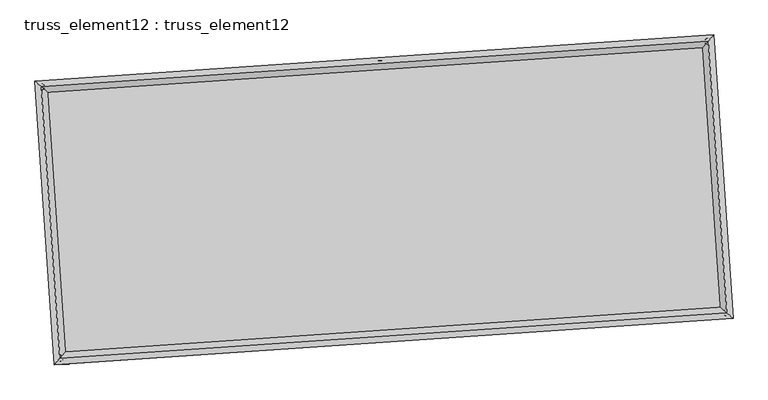
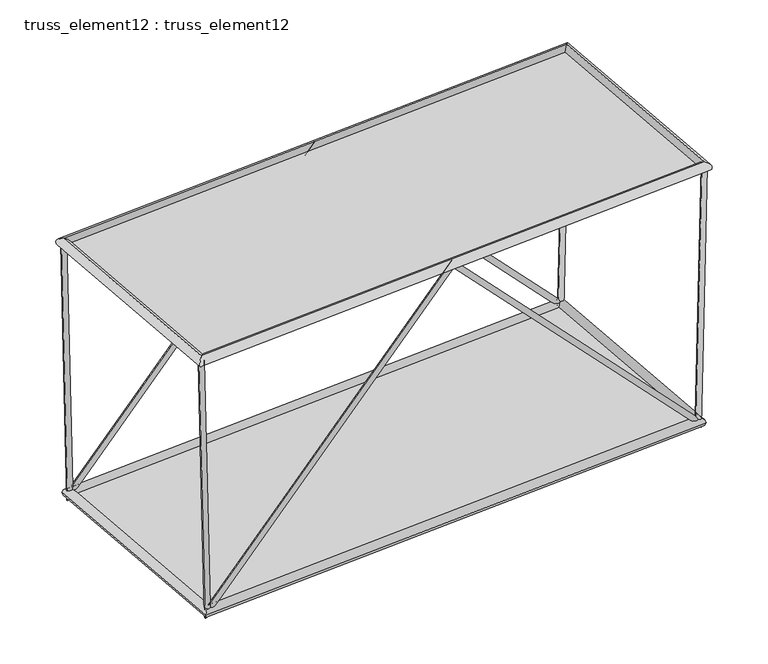
"""IFC4 building model written with IfcOpenShell, lengths in millimetres: plate geometry, truss_element12 : truss_element12."""

from ifc_helpers import new_model, si_unit, frame, origin, origin_with_axes, place, context, project, spatial, polyline, circle_curve, ellipse_curve, outline, extrude, source, transform, mapped, element, save
from ifc_brep_helpers import plane_surface, cylinder_surface, advanced_brep


def truss_element12_truss_element12_a892e973(model_context):
    return source(origin(), model_context, "Body", "SolidModel", [
        advanced_brep(
        [(-3781.9001647, 2268.2490038, 4999.7954617), (-3880.9761734, 2254.8896434, 4997.4562298), (-3667.764278, 2276.0314961, 121.2292813), (-3761.2226048, 2263.055184, -121.2292813), (1063.7843207, 2598.6578087, 5070.7379408), (1064.2315522, 2592.0845597, 4926.5107211), (5795.2062001, 2921.2754808, 121.228402), (5889.5547769, 2921.1050077, -121.228402), (5909.4678674, 2929.0665496, 4999.7937205), (6009.4402165, 2929.2795401, 4997.4519118)],
        [
            (0, 1, circle_curve(frame((-3831.4381691, 2261.5693236, 4998.6258457), z_axis=(-0.02338894552682542, -0.0015948032857686179, 0.9997251691488132), x_axis=(-0.13359419431199426, 0.9910349164502389, -0.0015445460813113196)), 50.0)),
            (1, 0, circle_curve(frame((-3831.4381691, 2261.5693236, 4998.6258457), z_axis=(-0.02338894552682542, -0.0015948032857686179, 0.9997251691488132), x_axis=(-0.13359419431199426, 0.9910349164502389, -0.0015445460813113196)), 50.0)),
            (0, 2),
            (2, 3, ellipse_curve(frame((-3714.4934414, 2269.54334, 0.0), z_axis=(-0.9300590534640556, -0.06341719137026212, 0.36189558840672914), x_axis=(0.3610572196661413, 0.024619119302049103, 0.9322186348125354)), 130.3269965, 50.0)),
            (3, 1),
            (3, 2, ellipse_curve(frame((-3714.4934414, 2269.54334, 0.0), z_axis=(-0.9300590534640556, -0.06341719137026212, 0.36189558840672914), x_axis=(0.3610572196661413, 0.024619119302049103, 0.9322186348125354)), 130.3269965, 50.0)),
            (2, 4),
            (4, 5, ellipse_curve(frame((1064.0079364, 2595.3711842, 4998.6243309), z_axis=(-0.997683396052257, -0.06802823822715924, 6.733807032577008e-06), x_axis=(-6.718207468772972e-06, -4.580890289962869e-07, -0.9999999999773278)), 72.2706352, 50.0)),
            (5, 3),
            (5, 4, ellipse_curve(frame((1064.0079364, 2595.3711842, 4998.6243309), z_axis=(-0.997683396052257, -0.06802823822715924, 6.733807032577008e-06), x_axis=(-6.718207468772972e-06, -4.580890289962869e-07, -0.9999999999773278)), 72.2706352, 50.0)),
            (4, 6),
            (6, 7, ellipse_curve(frame((5842.3804885, 2921.1902443, 0.0), z_axis=(-0.9300661480063922, -0.06341767512013534, -0.3618772703761719), x_axis=(-0.3610389440712053, -0.024617873158702383, 0.9322257458282791)), 130.3250571, 50.0)),
            (7, 5),
            (7, 6, ellipse_curve(frame((5842.3804885, 2921.1902443, 0.0), z_axis=(-0.9300661480063922, -0.06341767512013534, -0.3618772703761719), x_axis=(-0.3610389440712053, -0.024617873158702383, 0.9322257458282791)), 130.3250571, 50.0)),
            (8, 9, circle_curve(frame((5959.4540419, 2929.1730448, 4998.6228161), z_axis=(0.02341471068854339, 0.0015965601142037436, 0.9997245632268789), x_axis=(-0.0021667064549673746, 0.9999964572445558, -0.0015462475466263355)), 50.0)),
            (9, 8, circle_curve(frame((5959.4540419, 2929.1730448, 4998.6228161), z_axis=(0.02341471068854339, 0.0015965601142037436, 0.9997245632268789), x_axis=(-0.0021667064549673746, 0.9999964572445558, -0.0015462475466263355)), 50.0)),
            (6, 8),
            (9, 7),
        ],
        [
            plane_surface(frame((-3831.4381691, 2311.56926, 4998.7056077), z_axis=(-0.023388945526825605, -0.0015948032857737312, 0.9997251691488132), x_axis=(0.9997264411963621, -3.731097392201122e-05, 0.023388915766833666))),
            cylinder_surface(frame((-3831.4381691, 2261.5693236, 4998.6258457), z_axis=(-0.02338894552682542, -0.0015948032857686179, 0.9997251691488132), x_axis=(-0.13359419431199426, 0.9910349164502389, -0.0015445460813113196)), 50.0),
            cylinder_surface(frame((-3714.4934414, 2269.54334, 0.0), z_axis=(-0.6902460485200175, -0.04706525417770467, -0.7220424186650602), x_axis=(-0.0204192616913266, 0.9987518848874466, -0.04558208184971222)), 50.0),
            cylinder_surface(frame((1064.0079364, 2595.3711842, 4998.6243309), z_axis=(-0.6902363467958805, -0.04706459265401546, 0.7220517361520492), x_axis=(-0.11534221170273892, 0.9922794497620825, -0.045581441172688954)), 50.0),
            plane_surface(frame((5959.4540419, 2879.1731086, 4998.702666), z_axis=(0.02341471068854475, 0.0015965601141989436, 0.999724563226879), x_axis=(0.9997258380793066, -3.739324497509243e-05, -0.023414680830057922))),
            cylinder_surface(frame((5842.3804885, 2921.1902443, 0.0), z_axis=(-0.02341471068854339, -0.0015965601142037436, -0.9997245632268789), x_axis=(-0.0021667064549673746, 0.9999964572445558, -0.0015462475466263355)), 50.0),
        ],
        [
            (0, [[1, 2]]),
            (1, [[-1, 3, 4, 5]]),
            (1, [[-2, -5, 6, -3]]),
            (2, [[-4, 7, 8, 9]]),
            (2, [[-6, -9, 10, -7]]),
            (3, [[-8, 11, 12, 13]]),
            (3, [[-10, -13, 14, -11]]),
            (4, [[15, 16]]),
            (5, [[-12, 17, -16, 18]]),
            (5, [[-14, -18, -15, -17]]),
        ],
    ),
        advanced_brep(
        [(-3509.7872118, -1722.4845805, 4999.7954617), (-3608.8632204, -1735.8439409, 4997.4562298), (-3395.6513251, -1714.7020882, 121.2292813), (-3489.1096519, -1727.6784003, -121.2292813), (1335.8972737, -1392.0757756, 5070.7379408), (1336.3445051, -1398.6490246, 4926.5107211), (6067.319153, -1069.4581035, 121.228402), (6161.6677299, -1069.6285766, -121.228402), (6181.5808204, -1061.6670347, 4999.7937205), (6281.5531694, -1061.4540442, 4997.4519118)],
        [
            (0, 1, circle_curve(frame((-3559.3252161, -1729.1642607, 4998.6258457), z_axis=(-0.023388945526825546, -0.0015948032857685606, 0.9997251691488132), x_axis=(-0.1335941943119938, 0.991034916450239, -0.0015445460813113816)), 50.0)),
            (1, 0, circle_curve(frame((-3559.3252161, -1729.1642607, 4998.6258457), z_axis=(-0.023388945526825546, -0.0015948032857685606, 0.9997251691488132), x_axis=(-0.1335941943119938, 0.991034916450239, -0.0015445460813113816)), 50.0)),
            (0, 2),
            (2, 3, ellipse_curve(frame((-3442.3804885, -1721.1902443, 0.0), z_axis=(-0.9300590534640557, -0.06341719137026187, 0.36189558840672914), x_axis=(0.36105721966614135, 0.024619119302049068, 0.9322186348125354)), 130.3269965, 50.0)),
            (3, 1),
            (3, 2, ellipse_curve(frame((-3442.3804885, -1721.1902443, 0.0), z_axis=(-0.9300590534640557, -0.06341719137026187, 0.36189558840672914), x_axis=(0.36105721966614135, 0.024619119302049068, 0.9322186348125354)), 130.3269965, 50.0)),
            (2, 4),
            (4, 5, ellipse_curve(frame((1336.1208894, -1395.3624001, 4998.6243309), z_axis=(-0.997683396052257, -0.06802823822715906, 6.733807032737481e-06), x_axis=(-6.718207468926731e-06, -4.580890289866768e-07, -0.9999999999773278)), 72.2706352, 50.0)),
            (5, 3),
            (5, 4, ellipse_curve(frame((1336.1208894, -1395.3624001, 4998.6243309), z_axis=(-0.997683396052257, -0.06802823822715906, 6.733807032737481e-06), x_axis=(-6.718207468926731e-06, -4.580890289866768e-07, -0.9999999999773278)), 72.2706352, 50.0)),
            (4, 6),
            (6, 7, ellipse_curve(frame((6114.4934414, -1069.54334, 0.0), z_axis=(-0.9300661480063922, -0.06341767512013499, -0.36187727037617134), x_axis=(-0.36103894407120507, -0.024617873158702393, 0.9322257458282792)), 130.3250571, 50.0)),
            (7, 5),
            (7, 6, ellipse_curve(frame((6114.4934414, -1069.54334, 0.0), z_axis=(-0.9300661480063922, -0.06341767512013499, -0.36187727037617134), x_axis=(-0.36103894407120507, -0.024617873158702393, 0.9322257458282792)), 130.3250571, 50.0)),
            (8, 9, circle_curve(frame((6231.5669949, -1061.5605395, 4998.6228161), z_axis=(0.023414710688543654, 0.0015965601142036118, 0.9997245632268787), x_axis=(-0.002166706454967089, 0.9999964572445559, -0.0015462475466262102)), 50.0)),
            (9, 8, circle_curve(frame((6231.5669949, -1061.5605395, 4998.6228161), z_axis=(0.023414710688543654, 0.0015965601142036118, 0.9997245632268787), x_axis=(-0.002166706454967089, 0.9999964572445559, -0.0015462475466262102)), 50.0)),
            (6, 8),
            (9, 7),
        ],
        [
            plane_surface(frame((-3559.3252161, -1679.1643243, 4998.7056077), z_axis=(-0.023388945526825605, -0.0015948032857737268, 0.9997251691488132), x_axis=(0.9997264411963621, -3.731097392201122e-05, 0.023388915766833666))),
            cylinder_surface(frame((-3559.3252161, -1729.1642607, 4998.6258457), z_axis=(-0.023388945526825546, -0.0015948032857685606, 0.9997251691488132), x_axis=(-0.1335941943119938, 0.991034916450239, -0.0015445460813113816)), 50.0),
            cylinder_surface(frame((-3442.3804885, -1721.1902443, 0.0), z_axis=(-0.6902460485200175, -0.04706525417770453, -0.7220424186650602), x_axis=(-0.020419261691326598, 0.9987518848874467, -0.04558208184971204)), 50.0),
            cylinder_surface(frame((1336.1208894, -1395.3624001, 4998.6243309), z_axis=(-0.6902363467958806, -0.047064592654015365, 0.7220517361520495), x_axis=(-0.11534221170273865, 0.9922794497620827, -0.0455814411726888)), 50.0),
            plane_surface(frame((6231.5669949, -1111.5604757, 4998.702666), z_axis=(0.02341471068854475, 0.0015965601141989436, 0.999724563226879), x_axis=(0.9997258380793066, -3.739324497464834e-05, -0.023414680830057922))),
            cylinder_surface(frame((6114.4934414, -1069.54334, 0.0), z_axis=(-0.023414710688543658, -0.0015965601142036122, -0.999724563226879), x_axis=(-0.002166706454967089, 0.9999964572445559, -0.0015462475466262102)), 50.0),
        ],
        [
            (0, [[1, 2]]),
            (1, [[-1, 3, 4, 5]]),
            (1, [[-2, -5, 6, -3]]),
            (2, [[-4, 7, 8, 9]]),
            (2, [[-6, -9, 10, -7]]),
            (3, [[-8, 11, 12, 13]]),
            (3, [[-10, -13, 14, -11]]),
            (4, [[15, 16]]),
            (5, [[-12, 17, -16, 18]]),
            (5, [[-14, -18, -15, -17]]),
        ],
    ),
        advanced_brep(
        [(-3559.3260024, -1729.1651321, 4908.6258457), (-3559.3244299, -1729.1633893, 5088.6258457), (-3831.4372718, 2261.568567, 5088.6258457), (-3831.4390663, 2261.5700802, 4908.6258457), (5959.4533112, 2929.1721772, 5088.6228161), (5959.4547727, 2929.1739124, 4908.6228161), (6231.5661531, -1061.5597791, 5088.6228161), (6231.5678367, -1061.5612999, 4908.6228161)],
        [
            (0, 1, ellipse_curve(frame((-3559.3252161, -1729.1642607, 4998.6258457), z_axis=(-0.7535719234054201, 0.6573654662780878, 2.1829417809630158e-07), x_axis=(-0.6573654662780518, -0.7535719234054518, 2.182941780963455e-07)), 127.2792206, 90.0)),
            (1, 2),
            (2, 3, ellipse_curve(frame((-3831.4381691, 2261.5693236, 4998.6258457), z_axis=(-0.6573654662780518, -0.7535719234054514, 2.1829417809638662e-07), x_axis=(0.7535719234054199, -0.6573654662780882, -2.1829417809634269e-07)), 127.2792206, 90.0)),
            (3, 0),
            (1, 0, ellipse_curve(frame((-3559.3252161, -1729.1642607, 4998.6258457), z_axis=(-0.7535719234054201, 0.6573654662780878, 2.1829417809630158e-07), x_axis=(-0.6573654662780518, -0.7535719234054518, 2.182941780963455e-07)), 127.2792206, 90.0)),
            (3, 2, ellipse_curve(frame((-3831.4381691, 2261.5693236, 4998.6258457), z_axis=(-0.6573654662780518, -0.7535719234054514, 2.1829417809638662e-07), x_axis=(0.7535719234054199, -0.6573654662780882, -2.1829417809634269e-07)), 127.2792206, 90.0)),
            (2, 4),
            (4, 5, ellipse_curve(frame((5959.4540419, 2929.1730448, 4998.6228161), z_axis=(-0.7535719234054205, 0.6573654662780875, 2.1829417809638398e-07), x_axis=(-0.6573654662780517, -0.7535719234054518, 2.182941780963455e-07)), 127.2792206, 90.0)),
            (5, 3),
            (5, 4, ellipse_curve(frame((5959.4540419, 2929.1730448, 4998.6228161), z_axis=(-0.7535719234054205, 0.6573654662780875, 2.1829417809638398e-07), x_axis=(-0.6573654662780517, -0.7535719234054518, 2.182941780963455e-07)), 127.2792206, 90.0)),
            (4, 6),
            (6, 7, ellipse_curve(frame((6231.5669949, -1061.5605395, 4998.6228161), z_axis=(0.6573654662780518, 0.7535719234054516, -2.182941780963044e-07), x_axis=(-0.7535719234054203, 0.6573654662780877, 2.1829417809634276e-07)), 127.2792206, 90.0)),
            (7, 5),
            (7, 6, ellipse_curve(frame((6231.5669949, -1061.5605395, 4998.6228161), z_axis=(0.6573654662780518, 0.7535719234054516, -2.182941780963044e-07), x_axis=(-0.7535719234054203, 0.6573654662780877, 2.1829417809634276e-07)), 127.2792206, 90.0)),
            (6, 1),
            (0, 7),
        ],
        [
            cylinder_surface(frame((-3559.3252161, -1729.1642607, 4998.6258457), z_axis=(0.068028238228695, -0.997683396074877, 0.0), x_axis=(-0.9976833960310403, -0.06802823822570593, 9.37427355396154e-06)), 90.0),
            cylinder_surface(frame((-3831.4381691, 2261.5693236, 4998.6258457), z_axis=(-0.9976833960748295, -0.06802823822869196, 3.0871458725096684e-07), x_axis=(-0.06802823822310758, 0.9976833960340704, 9.065558966723289e-06)), 90.0),
            cylinder_surface(frame((5959.4540419, 2929.1730448, 4998.6228161), z_axis=(-0.06802823822869553, 0.9976833960748772, 0.0), x_axis=(0.9976833960366247, 0.06802823822608724, 8.75684437948504e-06)), 90.0),
            cylinder_surface(frame((6231.5669949, -1061.5605395, 4998.6228161), z_axis=(0.9976833960748296, 0.06802823822869167, -3.0871458725090866e-07), x_axis=(0.06802823822869167, -0.9976833960336897, 9.065558966723292e-06)), 90.0),
        ],
        [
            (0, [[1, 2, 3, 4]]),
            (0, [[5, -4, 6, -2]]),
            (1, [[-3, 7, 8, 9]]),
            (1, [[-6, -9, 10, -7]]),
            (2, [[-8, 11, 12, 13]]),
            (2, [[-10, -13, 14, -11]]),
            (3, [[-12, 15, -1, 16]]),
            (3, [[-14, -16, -5, -15]]),
        ],
    ),
        advanced_brep(
        [(-3358.7115243, -1625.2761972, 0.0), (-3526.0494527, -1817.1042913, 0.0), (-3810.4074885, 2353.2123043, 0.0), (-3618.5793943, 2185.8743758, 0.0), (5926.0494527, 3017.1042913, 0.0), (5758.7115243, 2825.2761972, 0.0), (6210.4074885, -1153.2123043, 0.0), (6018.5793943, -985.8743758, 0.0)],
        [
            (0, 1, ellipse_curve(frame((-3442.3804885, -1721.1902443, 0.0), z_axis=(-0.7535719234054582, 0.6573654662780805, 0.0), x_axis=(-0.6573654662780803, -0.7535719234054584, 0.0)), 127.2792206, 90.0)),
            (1, 2),
            (2, 3, ellipse_curve(frame((-3714.4934414, 2269.54334, 0.0), z_axis=(-0.6573654662780803, -0.7535719234054584, 0.0), x_axis=(0.7535719234054584, -0.6573654662780801, 0.0)), 127.2792206, 90.0)),
            (3, 0),
            (1, 0, ellipse_curve(frame((-3442.3804885, -1721.1902443, 0.0), z_axis=(-0.7535719234054582, 0.6573654662780805, 0.0), x_axis=(-0.6573654662780803, -0.7535719234054584, 0.0)), 127.2792206, 90.0)),
            (3, 2, ellipse_curve(frame((-3714.4934414, 2269.54334, 0.0), z_axis=(-0.6573654662780803, -0.7535719234054584, 0.0), x_axis=(0.7535719234054584, -0.6573654662780801, 0.0)), 127.2792206, 90.0)),
            (2, 4),
            (4, 5, ellipse_curve(frame((5842.3804885, 2921.1902443, 0.0), z_axis=(-0.7535719234054583, 0.6573654662780803, 0.0), x_axis=(-0.6573654662780803, -0.7535719234054583, 0.0)), 127.2792206, 90.0)),
            (5, 3),
            (5, 4, ellipse_curve(frame((5842.3804885, 2921.1902443, 0.0), z_axis=(-0.7535719234054583, 0.6573654662780803, 0.0), x_axis=(-0.6573654662780803, -0.7535719234054583, 0.0)), 127.2792206, 90.0)),
            (4, 6),
            (6, 7, ellipse_curve(frame((6114.4934414, -1069.54334, 0.0), z_axis=(0.6573654662780806, 0.7535719234054582, 0.0), x_axis=(-0.7535719234054582, 0.6573654662780806, 0.0)), 127.2792206, 90.0)),
            (7, 5),
            (7, 6, ellipse_curve(frame((6114.4934414, -1069.54334, 0.0), z_axis=(0.6573654662780806, 0.7535719234054582, 0.0), x_axis=(-0.7535719234054582, 0.6573654662780806, 0.0)), 127.2792206, 90.0)),
            (6, 1),
            (0, 7),
        ],
        [
            cylinder_surface(frame((-3442.3804885, -1721.1902443, 0.0), z_axis=(0.06802823822870183, -0.9976833960748765, 0.0), x_axis=(-0.9976833960748765, -0.06802823822870183, 0.0)), 90.0),
            cylinder_surface(frame((-3714.4934414, 2269.54334, 0.0), z_axis=(-0.9976833960748765, -0.068028238228702, 0.0), x_axis=(-0.068028238228702, 0.9976833960748765, 0.0)), 90.0),
            cylinder_surface(frame((5842.3804885, 2921.1902443, 0.0), z_axis=(-0.06802823822870174, 0.9976833960748765, 0.0), x_axis=(0.9976833960748765, 0.06802823822870174, 0.0)), 90.0),
            cylinder_surface(frame((6114.4934414, -1069.54334, 0.0), z_axis=(0.9976833960748768, 0.06802823822870133, 0.0), x_axis=(0.06802823822870133, -0.9976833960748768, 0.0)), 90.0),
        ],
        [
            (0, [[1, 2, 3, 4]]),
            (0, [[5, -4, 6, -2]]),
            (1, [[-3, 7, 8, 9]]),
            (1, [[-6, -9, 10, -7]]),
            (2, [[-8, 11, 12, 13]]),
            (2, [[-10, -13, 14, -11]]),
            (3, [[-12, 15, -1, 16]]),
            (3, [[-14, -16, -5, -15]]),
        ],
    ),
        extrude(outline(polyline([(-3442.3804885, -1721.1902443), (-3714.4934414, 2269.54334), (5842.3804885, 2921.1902443), (6114.4934414, -1069.54334), (-3442.3804885, -1721.1902443)])), origin_with_axes(), (0.0, 0.0, 1.0), 20.0),
        extrude(outline(polyline([(-2000.0000001, 4906.8132483), (2000.0, 4906.8132484), (2000.0, -4906.8132483), (-2000.0000001, -4906.8132484), (-2000.0000001, 4906.8132483)])), frame((1200.0644129, 600.0043921, 4998.6243309), z_axis=(3.0799941782636943e-07, 2.1001309486182012e-08, 0.9999999999999525), x_axis=(-0.06802823822870138, 0.9976833960748767, 0.0)), (0.0, 0.0, 1.0), 20.0),
    ])


if __name__ == "__main__":
    model = new_model("IFC4")
    model_context = context("Model", 3, world=origin())
    ifc_project = project(units=[si_unit("LENGTHUNIT", "METRE", prefix="MILLI")], contexts=[model_context])
    site = spatial("IfcSite", under=ifc_project)
    building = spatial("IfcBuilding", under=site)
    placement = place(None, origin())
    truss_element12_truss_element12_shape = truss_element12_truss_element12_a892e973(model_context)
    element("IfcPlate", 1, ObjectType="truss_element12 : truss_element12", at=placement, inside=building, context=model_context, shape_type="MappedRepresentation", body=[
        mapped(truss_element12_truss_element12_shape, transform((0.0, 0.0, 0.0), x_axis=(1.0, 0.0, 0.0), y_axis=(0.0, 1.0, 0.0), z_axis=(0.0, 0.0, 1.0))),
    ])
    save(model, "model.ifc")

# Revit data of these elements
# Type "truss_element12 : truss_element12"
#   steellbar1 = 90 mm
#   steelbar2 = 50 mm
#   offset1 = 5000 mm
#   M = Default Roof
# Element 1 (IfcPlate, "truss_element12 : truss_element12")
#   Materials on its faces: "Default Roof"
# Materials
#   "Default Roof": class "Miscellaneous", colour RGB 0 127 0, transparency 0, Comments = "Rendering appearance not upgraded Rendering appearance not upgraded ", Cost = 0
